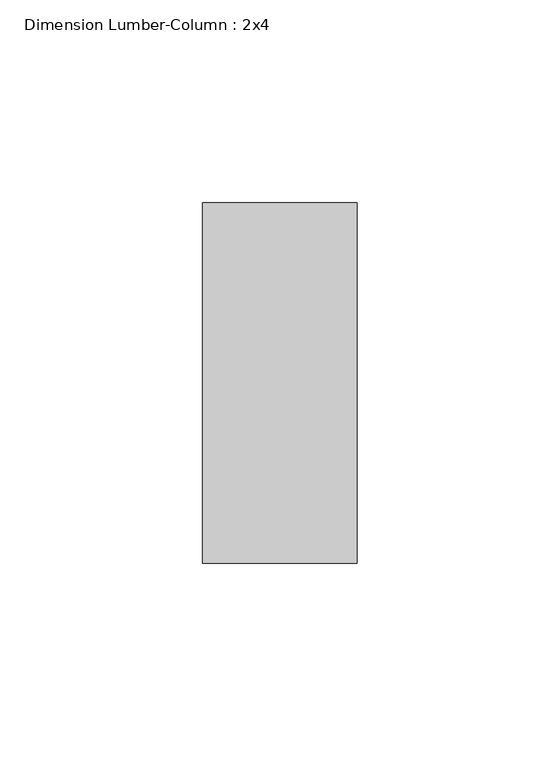
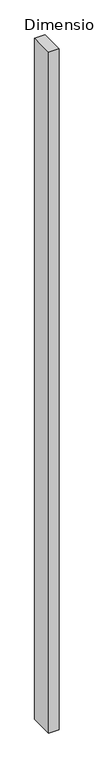
"""IFC4 building model written with IfcOpenShell, lengths in millimetres: column geometry, Dimension Lumber-Column : 2x4."""

from ifc_helpers import new_model, si_unit, frame, origin, place, context, project, spatial, polyline, outline, extrude, source, transform, mapped, element, save


def dimension_lumber_column_2x4_f24b5bbb(model_context):
    return source(origin(), model_context, "Body", "SweptSolid", [
        extrude(outline(polyline([(19.05, -44.45), (-19.05, -44.45), (-19.05, 44.45), (19.05, 44.45), (19.05, -44.45)])), frame((0.0, 0.0, 56.35625), z_axis=(0.0, 0.0, 1.0), x_axis=(1.0, 0.0, 0.0)), (0.0, 0.0, 1.0), 2636.04375),
    ])


if __name__ == "__main__":
    model = new_model("IFC4")
    model_context = context("Model", 3, world=origin())
    ifc_project = project(units=[si_unit("LENGTHUNIT", "METRE", prefix="MILLI")], contexts=[model_context])
    site = spatial("IfcSite", under=ifc_project)
    building = spatial("IfcBuilding", under=site)
    placement = place(None, origin())
    dimension_lumber_column_2x4_shape = dimension_lumber_column_2x4_f24b5bbb(model_context)
    element("IfcColumn", 1, ObjectType="Dimension Lumber-Column : 2x4", at=placement, inside=building, context=model_context, shape_type="MappedRepresentation", body=[
        mapped(dimension_lumber_column_2x4_shape, transform((0.0, 0.0, 0.0), x_axis=(1.0, 0.0, 0.0), y_axis=(0.0, 1.0, 0.0), z_axis=(0.0, 0.0, 1.0))),
    ])
    save(model, "model.ifc")

# Revit data of these elements
# Type "Dimension Lumber-Column : 2x4"
#   Int Type = "Interior"
#   Assembly Code = "B10"
#   Cost = 8.05
#   A = 0.0364583 SF
#   b = 0' - 1 1/2"
#   d = 0' - 3 1/2"
#   Structural Material [instance default] = Softwood, Lumber
# Element 1 (IfcColumn, "Dimension Lumber-Column : 2x4")
#   Structural Material = Douglas Fir #2
#   Materials on its faces: "Douglas Fir #2"
# Materials
#   "Softwood, Lumber": class "Wood", colour RGB 223 192 134, transparency 0, Description = "Pinus Echinata", Cost = 0
#   "Douglas Fir #2": class "Wood", colour RGB 223 192 134, transparency 0, Description = "Pinus Echinata", Cost = 0
